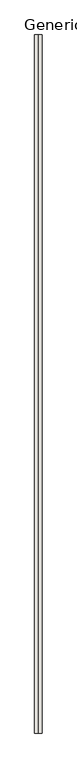
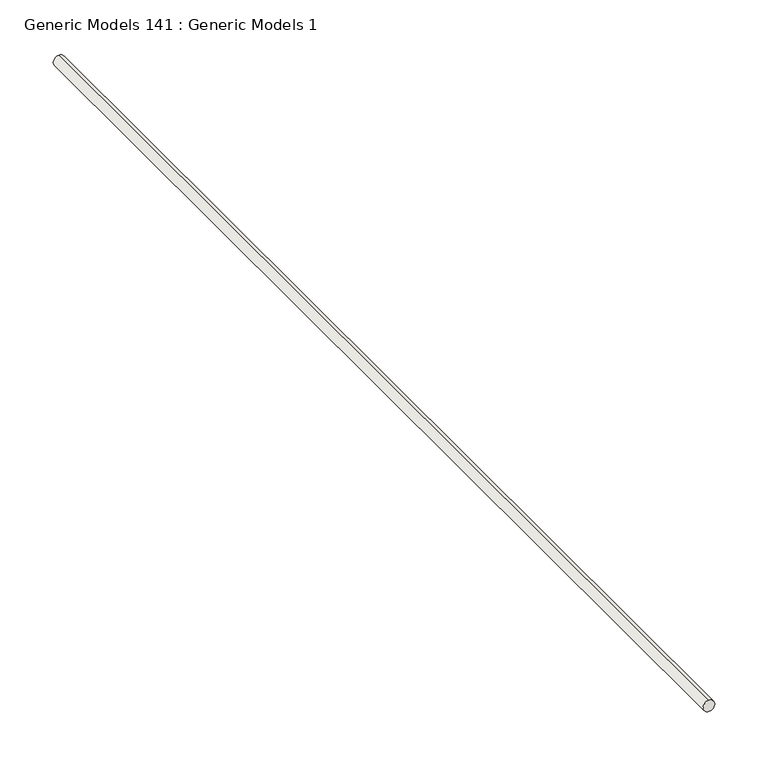
"""IFC4 building model written with IfcOpenShell, lengths in millimetres: wall geometry, Generic Models 141 : Generic Models 1."""

from ifc_helpers import new_model, si_unit, point, frame, frame_2d, origin, place, context, project, spatial, circle_curve, trimmed, segment, composite_curve, outline, extrude, source, transform, mapped, element, save


def generic_models_141_generic_models_1_1dd9f353(model_context):
    return source(origin(), model_context, "Body", "SweptSolid", [
        extrude(outline(composite_curve([segment(trimmed(circle_curve(frame_2d((-381.0, 51947.7625)), 6.35), [point((-374.65, 51947.7625))], [point((-387.35, 51947.7625))], False, "CARTESIAN"), True, "CONTINUOUS"), segment(trimmed(circle_curve(frame_2d((-381.0, 51947.7625)), 6.35), [point((-387.35, 51947.7625))], [point((-374.65, 51947.7625))], False, "CARTESIAN"), True, "CONTINUOUS")], self_intersect=False)), frame((0.0, 0.0, 0.0), z_axis=(0.0, 1.0, 0.0), x_axis=(0.0, 0.0, 1.0)), (0.0, 0.0, 1.0), 1219.2),
    ])


if __name__ == "__main__":
    model = new_model("IFC4")
    model_context = context("Model", 3, world=origin())
    ifc_project = project(units=[si_unit("LENGTHUNIT", "METRE", prefix="MILLI")], contexts=[model_context])
    site = spatial("IfcSite", under=ifc_project)
    building = spatial("IfcBuilding", under=site)
    placement = place(None, origin())
    generic_models_141_generic_models_1_shape = generic_models_141_generic_models_1_1dd9f353(model_context)
    element("IfcWall", 1, ObjectType="Generic Models 141 : Generic Models 1", at=placement, inside=building, context=model_context, shape_type="MappedRepresentation", body=[
        mapped(generic_models_141_generic_models_1_shape, transform((0.0, 0.0, 0.0), x_axis=(1.0, 0.0, 0.0), y_axis=(0.0, 1.0, 0.0), z_axis=(0.0, 0.0, 1.0))),
    ])
    save(model, "model.ifc")

# Revit data of these elements
# Element 1 (IfcWall, "Generic Models 141 : Generic Models 1")
#   Materials on its faces: "#4 CONT. STEEL REBAR"
# Materials
#   "#4 CONT. STEEL REBAR": class "Metal", colour RGB 189 187 185, transparency 0, Description = "Structural steel 50ksi", Cost = 0
